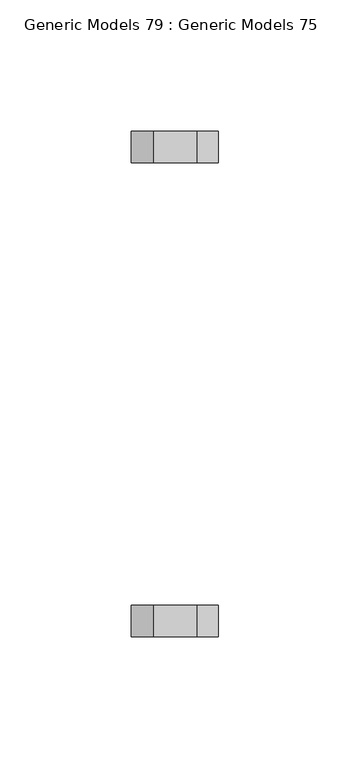
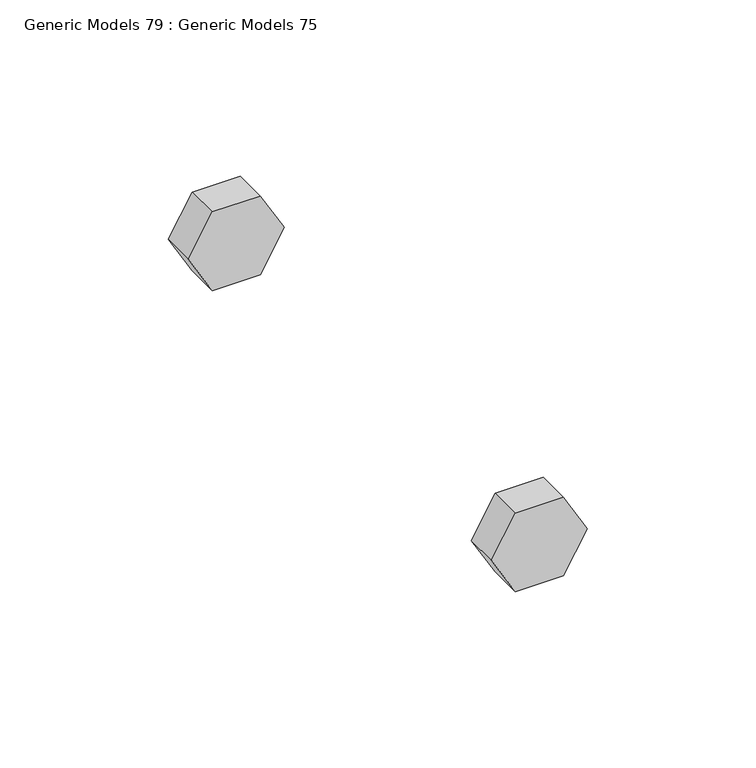
"""IFC4 building model written with IfcOpenShell, lengths in millimetres: proxy geometry, Generic Models 79 : Generic Models 75."""

from ifc_helpers import new_model, si_unit, frame, origin, place, context, project, spatial, polyline, outline, extrude, source, transform, mapped, element, save


def generic_models_79_generic_models_75_cd3e6485(model_context):
    return source(origin(), model_context, "Body", "SweptSolid", [
        extrude(outline(polyline([(271505.3625, 31979.8726858), (271505.3625, 31996.3704698), (271519.65, 32004.6193618), (271533.9375, 31996.3704698), (271533.9375, 31979.8726858), (271519.65, 31971.6237939), (271505.3625, 31979.8726858)])), frame((0.0, 36311.3770442, 0.0), z_axis=(0.0, 1.0, 0.0), x_axis=(0.0, 0.0, 1.0)), (0.0, 0.0, 1.0), 11.90625),
        extrude(outline(polyline([(271505.3625, 31979.8726858), (271505.3625, 31996.3704698), (271519.65, 32004.6193618), (271533.9375, 31996.3704698), (271533.9375, 31979.8726858), (271519.65, 31971.6237939), (271505.3625, 31979.8726858)])), frame((0.0, 36491.5582942, 0.0), z_axis=(0.0, 1.0, 0.0), x_axis=(0.0, 0.0, 1.0)), (0.0, 0.0, 1.0), 11.90625),
    ])


if __name__ == "__main__":
    model = new_model("IFC4")
    model_context = context("Model", 3, world=origin())
    ifc_project = project(units=[si_unit("LENGTHUNIT", "METRE", prefix="MILLI")], contexts=[model_context])
    site = spatial("IfcSite", under=ifc_project)
    building = spatial("IfcBuilding", under=site)
    placement = place(None, origin())
    generic_models_79_generic_models_75_shape = generic_models_79_generic_models_75_cd3e6485(model_context)
    element("IfcBuildingElementProxy", 1, Name="Generic Models 79 : Generic Models 75", ObjectType="Generic Models 79 : Generic Models 75", at=placement, inside=building, context=model_context, shape_type="MappedRepresentation", body=[
        mapped(generic_models_79_generic_models_75_shape, transform((0.0, 0.0, 0.0), x_axis=(1.0, 0.0, 0.0), y_axis=(0.0, 1.0, 0.0), z_axis=(0.0, 0.0, 1.0))),
    ])
    save(model, "model.ifc")

# Revit data of these elements
# Element 1 (IfcBuildingElementProxy, "Generic Models 79 : Generic Models 75")
#   Materials on its faces: "3/4\" GALV. THRU BOLTS"
# Materials
#   "3/4\" GALV. THRU BOLTS": class "Generic", colour RGB 105 69 171, transparency 0, Cost = 0
